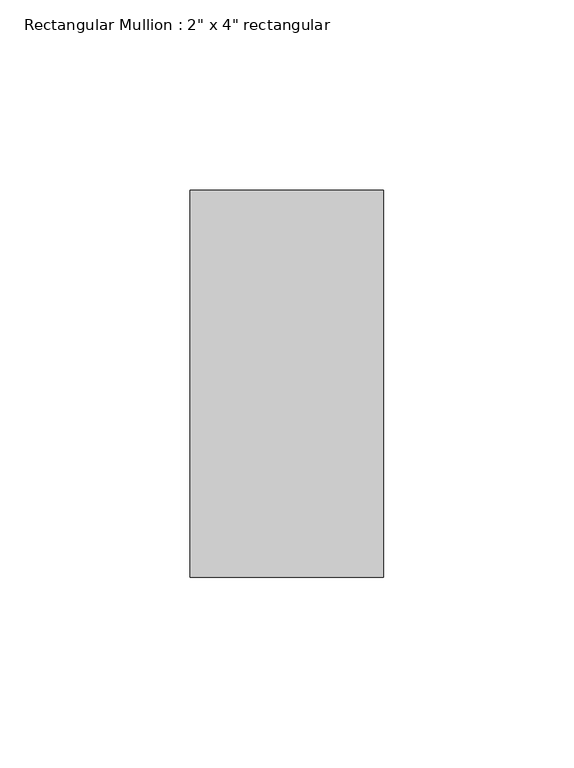
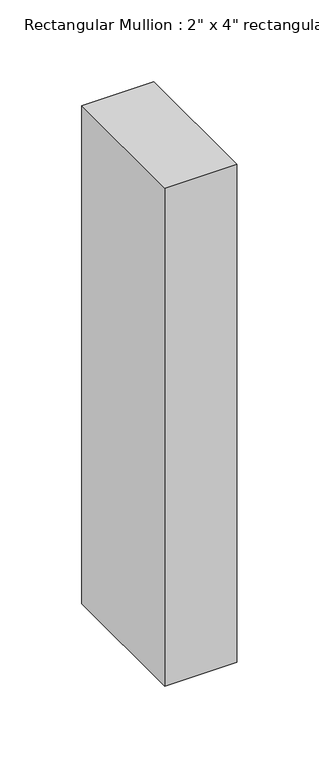
"""IFC4 building model written with IfcOpenShell, lengths in millimetres: member geometry."""

from ifc_helpers import new_model, si_unit, frame, origin, place, context, project, spatial, polyline, outline, extrude, source, transform, mapped, element, save


def member_6ec70098(model_context):
    return source(origin(), model_context, "Body", "SweptSolid", [
        extrude(outline(polyline([(25.4, 50.8), (25.4, -50.8), (-25.4, -50.8), (-25.4, 50.8), (25.4, 50.8)])), frame((0.0, 0.0, -371.9285714), z_axis=(0.0, 0.0, 1.0), x_axis=(1.0, 0.0, 0.0)), (0.0, 0.0, 1.0), 371.9285714),
    ])


if __name__ == "__main__":
    model = new_model("IFC4")
    model_context = context("Model", 3, world=origin())
    ifc_project = project(units=[si_unit("LENGTHUNIT", "METRE", prefix="MILLI")], contexts=[model_context])
    site = spatial("IfcSite", under=ifc_project)
    building = spatial("IfcBuilding", under=site)
    placement = place(None, origin())
    member_shape = member_6ec70098(model_context)
    element("IfcMember", 1, ObjectType="Rectangular Mullion : 2\" x 4\" rectangular", at=placement, inside=building, context=model_context, shape_type="MappedRepresentation", body=[
        mapped(member_shape, transform((0.0, 0.0, 0.0), x_axis=(1.0, 0.0, 0.0), y_axis=(0.0, 1.0, 0.0), z_axis=(0.0, 0.0, 1.0))),
    ])
    save(model, "model.ifc")

# Revit data of these elements
# Type "Rectangular Mullion : 2\" x 4\" rectangular"
#   built-in parameter 1007304 = 0.333333 (stored number, unit not read)
#   built-in parameter 1007301 = 0.0833333 (stored number, unit not read)
#   built-in parameter 1007300 = 0.0833333 (stored number, unit not read)
